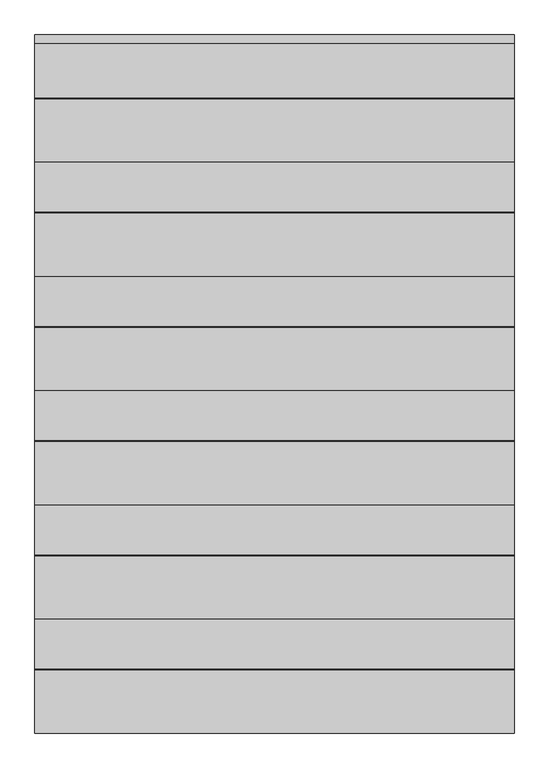
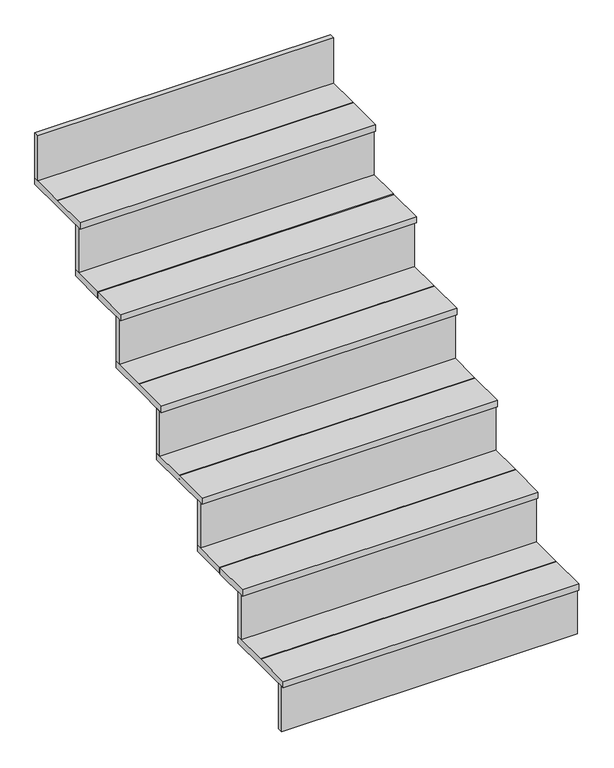
"""IFC4 building model written with IfcOpenShell, lengths in millimetres: stair flight geometry."""

from ifc_helpers import new_model, si_unit, frame, origin, origin_with_axes, place, context, project, spatial, polyline, outline, extrude, source, transform, mapped, element, save


def stair_flight_a84faa77(model_context):
    return source(origin(), model_context, "Body", "SweptSolid", [
        extrude(outline(polyline([(-21616.6414763, -10959.3570712), (-21616.6414763, -10978.4070712), (-22683.4414763, -10978.4070712), (-22683.4414763, -10959.3570712), (-21616.6414763, -10959.3570712)])), origin_with_axes(), (0.0, 0.0, 1.0), 172.0311384),
        extrude(outline(polyline([(-10848.2320712, 172.0311384), (-10987.9320712, 172.0311384), (-10987.9320712, 195.9428571), (-10848.2320712, 195.9428571), (-10848.2320712, 184.1885851), (-10845.0570712, 184.1885851), (-10845.0570712, 195.9428571), (-10705.3570712, 195.9428571), (-10705.3570712, 172.0311384), (-10845.0570712, 172.0311384), (-10845.0570712, 183.7854105), (-10848.2320712, 183.7854105), (-10848.2320712, 172.0311384)])), frame((-22683.4414763, 0.0, 0.0), z_axis=(1.0, 0.0, 0.0), x_axis=(0.0, 1.0, 0.0)), (0.0, 0.0, 1.0), 1066.8),
        extrude(outline(polyline([(-21616.6414763, -10705.3570712), (-21616.6414763, -10724.4070712), (-22683.4414763, -10724.4070712), (-22683.4414763, -10705.3570712), (-21616.6414763, -10705.3570712)])), frame((0.0, 0.0, 195.9428571), z_axis=(0.0, 0.0, 1.0), x_axis=(1.0, 0.0, 0.0)), (0.0, 0.0, 1.0), 172.0311384),
        extrude(outline(polyline([(-10594.2320712, 367.9739955), (-10733.9320712, 367.9739955), (-10733.9320712, 391.8857143), (-10594.2320712, 391.8857143), (-10594.2320712, 380.1314422), (-10591.0570712, 380.1314422), (-10591.0570712, 391.8857143), (-10451.3570712, 391.8857143), (-10451.3570712, 367.9739955), (-10591.0570712, 367.9739955), (-10591.0570712, 379.7282676), (-10594.2320712, 379.7282676), (-10594.2320712, 367.9739955)])), frame((-22683.4414763, 0.0, 0.0), z_axis=(1.0, 0.0, 0.0), x_axis=(0.0, 1.0, 0.0)), (0.0, 0.0, 1.0), 1066.8),
        extrude(outline(polyline([(-21616.6414763, -10451.3570712), (-21616.6414763, -10470.4070712), (-22683.4414763, -10470.4070712), (-22683.4414763, -10451.3570712), (-21616.6414763, -10451.3570712)])), frame((0.0, 0.0, 391.8857143), z_axis=(0.0, 0.0, 1.0), x_axis=(1.0, 0.0, 0.0)), (0.0, 0.0, 1.0), 172.0311384),
        extrude(outline(polyline([(-10340.2320712, 563.9168527), (-10479.9320712, 563.9168527), (-10479.9320712, 587.8285714), (-10340.2320712, 587.8285714), (-10340.2320712, 576.0742994), (-10337.0570712, 576.0742994), (-10337.0570712, 587.8285714), (-10197.3570712, 587.8285714), (-10197.3570712, 563.9168527), (-10337.0570712, 563.9168527), (-10337.0570712, 575.6711248), (-10340.2320712, 575.6711248), (-10340.2320712, 563.9168527)])), frame((-22683.4414763, 0.0, 0.0), z_axis=(1.0, 0.0, 0.0), x_axis=(0.0, 1.0, 0.0)), (0.0, 0.0, 1.0), 1066.8),
        extrude(outline(polyline([(-21616.6414763, -10197.3570712), (-21616.6414763, -10216.4070712), (-22683.4414763, -10216.4070712), (-22683.4414763, -10197.3570712), (-21616.6414763, -10197.3570712)])), frame((0.0, 0.0, 587.8285714), z_axis=(0.0, 0.0, 1.0), x_axis=(1.0, 0.0, 0.0)), (0.0, 0.0, 1.0), 172.0311384),
        extrude(outline(polyline([(-10086.2320712, 759.8597098), (-10225.9320712, 759.8597098), (-10225.9320712, 783.7714286), (-10086.2320712, 783.7714286), (-10086.2320712, 772.0171565), (-10083.0570712, 772.0171565), (-10083.0570712, 783.7714286), (-9943.3570712, 783.7714286), (-9943.3570712, 759.8597098), (-10083.0570712, 759.8597098), (-10083.0570712, 771.6139819), (-10086.2320712, 771.6139819), (-10086.2320712, 759.8597098)])), frame((-22683.4414763, 0.0, 0.0), z_axis=(1.0, 0.0, 0.0), x_axis=(0.0, 1.0, 0.0)), (0.0, 0.0, 1.0), 1066.8),
        extrude(outline(polyline([(-21616.6414763, -9943.3570712), (-21616.6414763, -9962.4070712), (-22683.4414763, -9962.4070712), (-22683.4414763, -9943.3570712), (-21616.6414763, -9943.3570712)])), frame((0.0, 0.0, 783.7714286), z_axis=(0.0, 0.0, 1.0), x_axis=(1.0, 0.0, 0.0)), (0.0, 0.0, 1.0), 172.0311384),
        extrude(outline(polyline([(-9832.2320712, 955.802567), (-9971.9320712, 955.802567), (-9971.9320712, 979.7142857), (-9832.2320712, 979.7142857), (-9832.2320712, 967.9600136), (-9829.0570712, 967.9600136), (-9829.0570712, 979.7142857), (-9689.3570712, 979.7142857), (-9689.3570712, 955.802567), (-9829.0570712, 955.802567), (-9829.0570712, 967.556839), (-9832.2320712, 967.556839), (-9832.2320712, 955.802567)])), frame((-22683.4414763, 0.0, 0.0), z_axis=(1.0, 0.0, 0.0), x_axis=(0.0, 1.0, 0.0)), (0.0, 0.0, 1.0), 1066.8),
        extrude(outline(polyline([(-21616.6414763, -9435.3570712), (-21616.6414763, -9454.4070712), (-22683.4414763, -9454.4070712), (-22683.4414763, -9435.3570712), (-21616.6414763, -9435.3570712)])), frame((0.0, 0.0, 1175.6571429), z_axis=(0.0, 0.0, 1.0), x_axis=(1.0, 0.0, 0.0)), (0.0, 0.0, 1.0), 172.0311384),
        extrude(outline(polyline([(-21616.6414763, -9689.3570712), (-21616.6414763, -9708.4070712), (-22683.4414763, -9708.4070712), (-22683.4414763, -9689.3570712), (-21616.6414763, -9689.3570712)])), frame((0.0, 0.0, 979.7142857), z_axis=(0.0, 0.0, 1.0), x_axis=(1.0, 0.0, 0.0)), (0.0, 0.0, 1.0), 172.0311384),
        extrude(outline(polyline([(-9578.2320712, 1151.7454241), (-9717.9320712, 1151.7454241), (-9717.9320712, 1175.6571429), (-9578.2320712, 1175.6571429), (-9578.2320712, 1163.9028708), (-9575.0570712, 1163.9028708), (-9575.0570712, 1175.6571429), (-9435.3570712, 1175.6571429), (-9435.3570712, 1151.7454241), (-9575.0570712, 1151.7454241), (-9575.0570712, 1163.4996962), (-9578.2320712, 1163.4996962), (-9578.2320712, 1151.7454241)])), frame((-22683.4414763, 0.0, 0.0), z_axis=(1.0, 0.0, 0.0), x_axis=(0.0, 1.0, 0.0)), (0.0, 0.0, 1.0), 1066.8),
    ])


if __name__ == "__main__":
    model = new_model("IFC4")
    model_context = context("Model", 3, world=origin())
    ifc_project = project(units=[si_unit("LENGTHUNIT", "METRE", prefix="MILLI")], contexts=[model_context])
    site = spatial("IfcSite", under=ifc_project)
    building = spatial("IfcBuilding", under=site)
    placement = place(None, origin())
    stair_flight_shape = stair_flight_a84faa77(model_context)
    element("IfcStairFlight", 1, at=placement, inside=building, context=model_context, shape_type="MappedRepresentation", body=[
        mapped(stair_flight_shape, transform((0.0, 0.0, 0.0), x_axis=(1.0, 0.0, 0.0), y_axis=(0.0, 1.0, 0.0), z_axis=(0.0, 0.0, 1.0))),
    ])
    save(model, "model.ifc")

# Revit data of these elements
# Element 1 (IfcStairFlight)
#   Materials on its faces: "Composite Deck - Trex - Select - 1x6 Square Edge Board - Saddle - 20'"
# Materials
#   "Composite Deck - Trex - Select - 1x6 Square Edge Board - Saddle - 20'": class "Wood", colour RGB 120 75 45, transparency 0, Keynote = "06 11 00", Model = "Trex Select® Composite Deck 1\" Square Edge Board", Manufacturer = "Trex", URL = "http://www.trex.com/", Description = "1x6 Trex Select® Composite Deck Square Edge Board", Cost = 0
